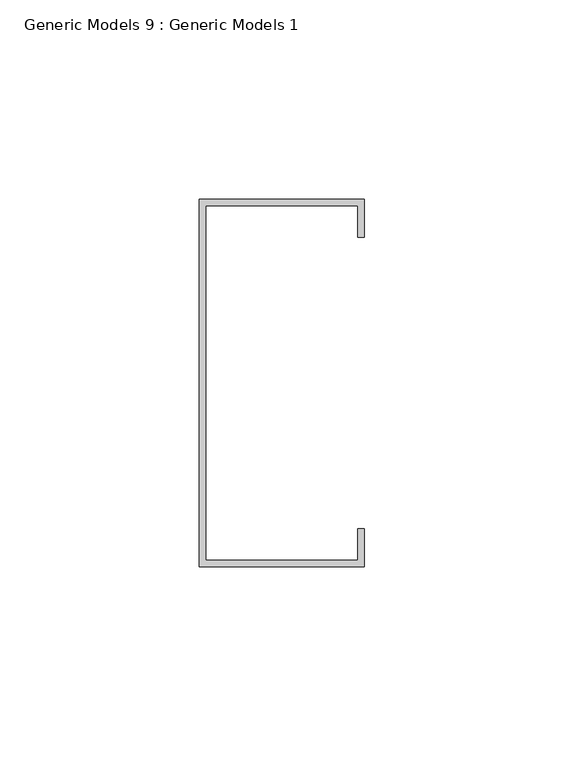
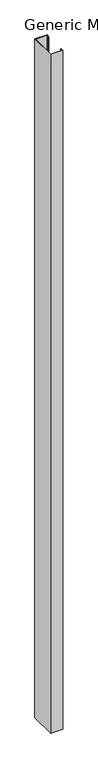
"""IFC4 building model written with IfcOpenShell, lengths in millimetres: proxy geometry, Generic Models 9 : Generic Models 1."""

from ifc_helpers import new_model, si_unit, frame, origin, place, context, project, spatial, polyline, outline, extrude, source, transform, mapped, element, save


def generic_models_9_generic_models_1_1d539265(model_context):
    return source(origin(), model_context, "Body", "SweptSolid", [
        extrude(outline(polyline([(14885.2842846, 5684.0157424), (14926.5592846, 5684.0157424), (14926.5592846, 5674.4907424), (14924.9717846, 5674.4907424), (14924.9717846, 5682.4282424), (14886.8717846, 5682.4282424), (14886.8717846, 5593.5282424), (14924.9717846, 5593.5282424), (14924.9717846, 5601.4657424), (14926.5592846, 5601.4657424), (14926.5592846, 5591.9407424), (14885.2842846, 5591.9407424), (14885.2842846, 5684.0157424)])), frame((0.0, 0.0, 450.7860265), z_axis=(0.0, 0.0, 1.0), x_axis=(1.0, 0.0, 0.0)), (0.0, 0.0, 1.0), 2438.4),
    ])


if __name__ == "__main__":
    model = new_model("IFC4")
    model_context = context("Model", 3, world=origin())
    ifc_project = project(units=[si_unit("LENGTHUNIT", "METRE", prefix="MILLI")], contexts=[model_context])
    site = spatial("IfcSite", under=ifc_project)
    building = spatial("IfcBuilding", under=site)
    placement = place(None, origin())
    generic_models_9_generic_models_1_shape = generic_models_9_generic_models_1_1d539265(model_context)
    element("IfcBuildingElementProxy", 1, Name="Generic Models 9 : Generic Models 1", ObjectType="Generic Models 9 : Generic Models 1", at=placement, inside=building, context=model_context, shape_type="MappedRepresentation", body=[
        mapped(generic_models_9_generic_models_1_shape, transform((0.0, 0.0, 0.0), x_axis=(1.0, 0.0, 0.0), y_axis=(0.0, 1.0, 0.0), z_axis=(0.0, 0.0, 1.0))),
    ])
    save(model, "model.ifc")

# Revit data of these elements
# Element 1 (IfcBuildingElementProxy, "Generic Models 9 : Generic Models 1")
#   Materials on its faces: "METAL STUDS"
# Materials
#   "METAL STUDS": class "Unassigned", colour RGB 210 209 208, transparency 0, Keynote = "M05121300.02", Cost = 0
